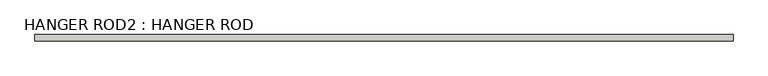
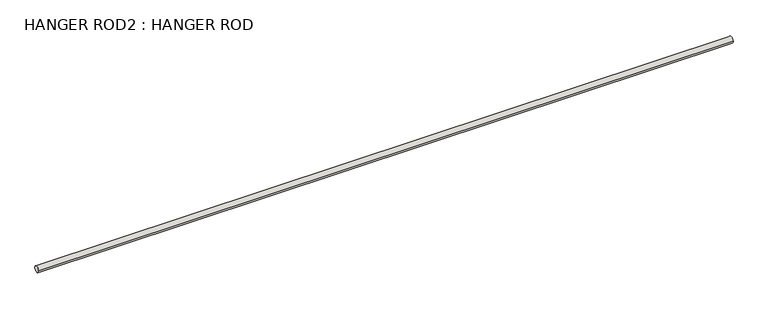
"""IFC4 building model written with IfcOpenShell, lengths in millimetres: wall geometry, HANGER ROD2 : HANGER ROD."""

from ifc_helpers import new_model, si_unit, point, frame, frame_2d, origin, place, context, project, spatial, circle_curve, trimmed, segment, composite_curve, outline, extrude, source, transform, mapped, element, save


def hanger_rod2_hanger_rod_ff50d585(model_context):
    return source(origin(), model_context, "Body", "SweptSolid", [
        extrude(outline(composite_curve([segment(trimmed(circle_curve(frame_2d((-1046.4884634, 4908.7706466)), 6.35), [point((-1040.1384634, 4908.7706466))], [point((-1052.8384634, 4908.7706466))], False, "CARTESIAN"), True, "CONTINUOUS"), segment(trimmed(circle_curve(frame_2d((-1046.4884634, 4908.7706466)), 6.35), [point((-1052.8384634, 4908.7706466))], [point((-1040.1384634, 4908.7706466))], False, "CARTESIAN"), True, "CONTINUOUS")], self_intersect=False)), frame((21459.3508034, 0.0, 0.0), z_axis=(1.0, 0.0, 0.0), x_axis=(0.0, 1.0, 0.0)), (0.0, 0.0, 1.0), 1405.2437091),
    ])


if __name__ == "__main__":
    model = new_model("IFC4")
    model_context = context("Model", 3, world=origin())
    ifc_project = project(units=[si_unit("LENGTHUNIT", "METRE", prefix="MILLI")], contexts=[model_context])
    site = spatial("IfcSite", under=ifc_project)
    building = spatial("IfcBuilding", under=site)
    placement = place(None, origin())
    hanger_rod2_hanger_rod_shape = hanger_rod2_hanger_rod_ff50d585(model_context)
    element("IfcWall", 1, ObjectType="HANGER ROD2 : HANGER ROD", at=placement, inside=building, context=model_context, shape_type="MappedRepresentation", body=[
        mapped(hanger_rod2_hanger_rod_shape, transform((0.0, 0.0, 0.0), x_axis=(1.0, 0.0, 0.0), y_axis=(0.0, 1.0, 0.0), z_axis=(0.0, 0.0, 1.0))),
    ])
    save(model, "model.ifc")

# Revit data of these elements
# Element 1 (IfcWall, "HANGER ROD2 : HANGER ROD")
#   Materials on its faces: "1/2\" STEEL ROD (RAW STEEL)"
# Materials
#   "1/2\" STEEL ROD (RAW STEEL)": class "Metal", colour RGB 189 187 185, transparency 0, Description = "Structural steel 50ksi", Cost = 0
